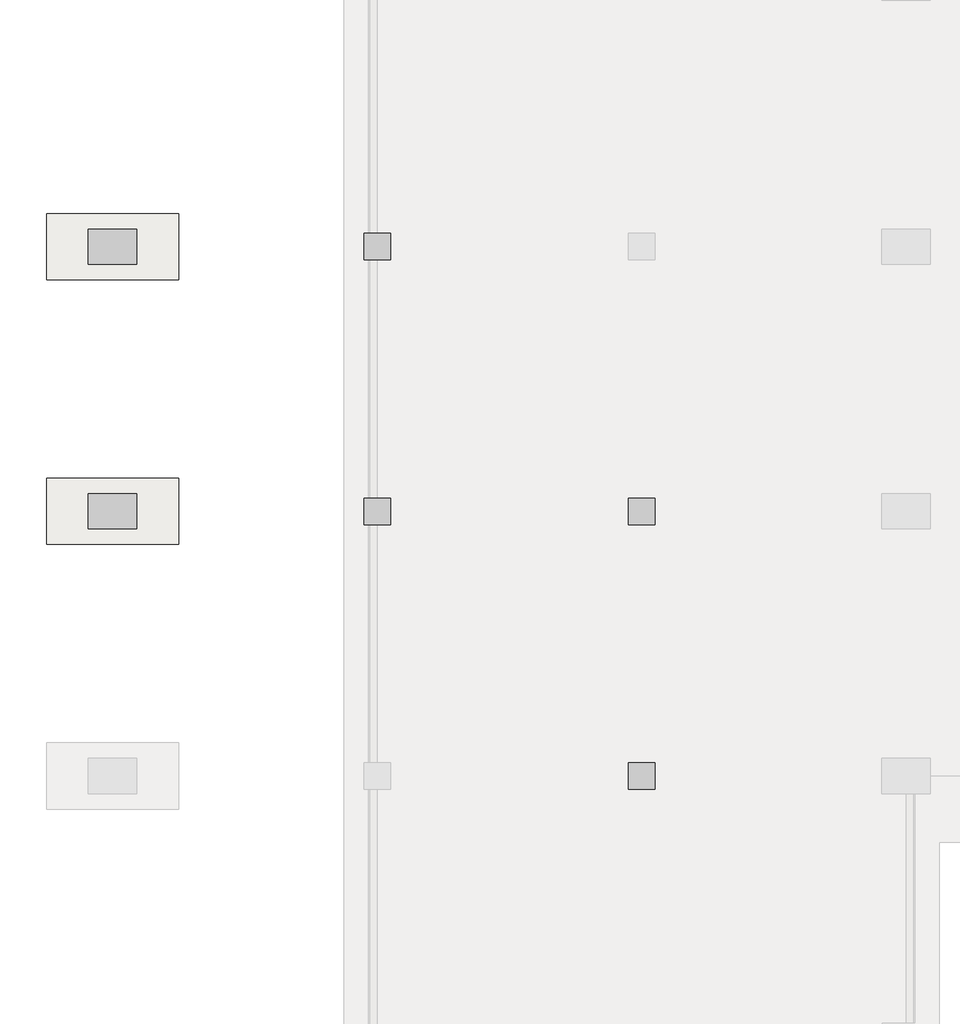
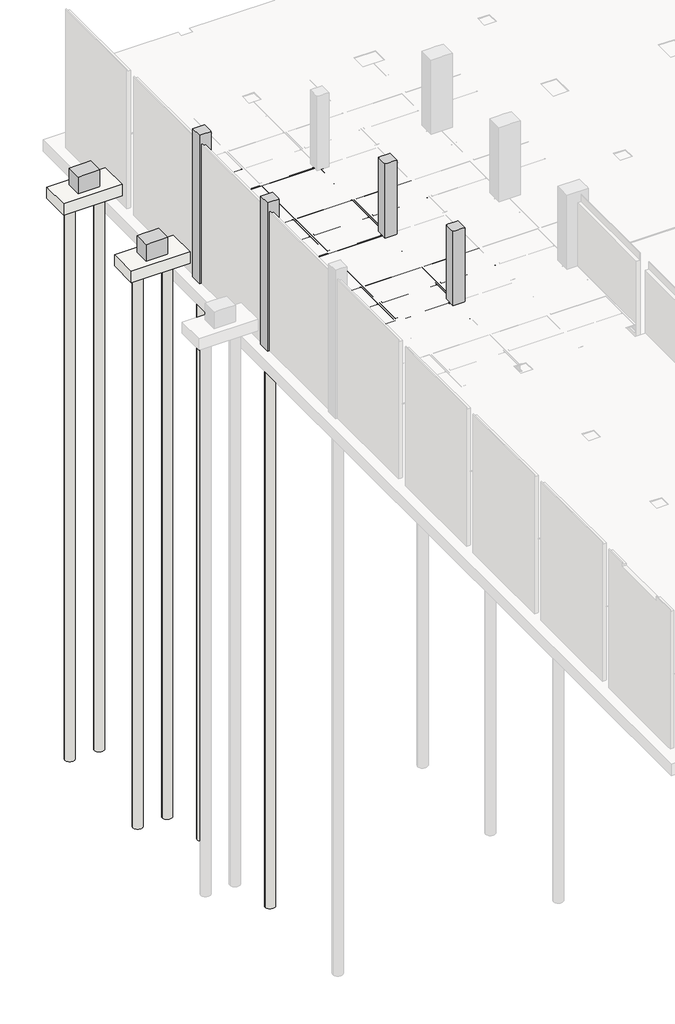
# Not in any storey, part 7 of 16: 27 beams, 8 slabs, 6 columns.
"""IFC4 building model written with IfcOpenShell, lengths in millimetres."""

from ifc_helpers import new_model, si_unit, point, frame, frame_2d, origin, place, context, project, spatial, polyline, circle_curve, trimmed, segment, composite_curve, outline, extrude, faceted_brep, element, save

model = new_model("IFC4")

# Units and contexts
model_context = context("Model", 3, world=origin())
ifc_project = project(units=[si_unit("LENGTHUNIT", "METRE", prefix="MILLI")], contexts=[model_context])

# Site, building
site = spatial("IfcSite", under=ifc_project)
building = spatial("IfcBuilding", under=site)

# Beams
placement = place(None, origin())
element("IfcBeam", 1, ObjectType="Steel Framing_H_KS : H_SB_AR_S02_H-400x200x8x13_BSG1", at=placement, inside=building, context=model_context, shape_type="SweptSolid", body=[
    extrude(outline(composite_curve([segment(polyline([(-17900.0, -4187.0381366), (-17900.0, -4200.0381366), (-18100.0, -4200.0381366), (-18100.0, -4187.0381366), (-18020.0, -4187.0381366)]), True, "CONTINUOUS"), segment(trimmed(circle_curve(frame_2d((-18020.0, -4171.0381366)), 16.0), [point((-18020.0, -4187.0381366))], [point((-18004.0, -4171.0381366))], True, "CARTESIAN"), True, "CONTINUOUS"), segment(polyline([(-18004.0, -4171.0381366), (-18004.0, -3829.0381366)]), True, "CONTINUOUS"), segment(trimmed(circle_curve(frame_2d((-18020.0, -3829.0381366)), 16.0), [point((-18004.0, -3829.0381366))], [point((-18020.0, -3813.0381366))], True, "CARTESIAN"), True, "CONTINUOUS"), segment(polyline([(-18020.0, -3813.0381366), (-18100.0, -3813.0381366), (-18100.0, -3800.0381366), (-17900.0, -3800.0381366), (-17900.0, -3813.0381366), (-17980.0, -3813.0381366)]), True, "CONTINUOUS"), segment(trimmed(circle_curve(frame_2d((-17980.0, -3829.0381366)), 16.0), [point((-17980.0, -3813.0381366))], [point((-17996.0, -3829.0381366))], True, "CARTESIAN"), True, "CONTINUOUS"), segment(polyline([(-17996.0, -3829.0381366), (-17996.0, -4171.0381366)]), True, "CONTINUOUS"), segment(trimmed(circle_curve(frame_2d((-17980.0, -4171.0381366)), 16.0), [point((-17996.0, -4171.0381366))], [point((-17980.0, -4187.0381366))], True, "CARTESIAN"), True, "CONTINUOUS"), segment(polyline([(-17980.0, -4187.0381366), (-17900.0, -4187.0381366)]), True, "CONTINUOUS")], self_intersect=False)), frame((24312.7, 0.0, 0.0), z_axis=(1.0, 0.0, 0.0), x_axis=(0.0, 1.0, 0.0)), (0.0, 0.0, 1.0), 5374.6),
])
element("IfcBeam", 2, ObjectType="Steel Framing_C_KS : H_SB_AR_S02_C-150x75x6.5x10_J1", at=placement, inside=building, context=model_context, shape_type="SweptSolid", body=[
    extrude(outline(composite_curve([segment(polyline([(-16477.2, -3800.0381366), (-16477.2, -3950.0381366), (-16552.2, -3950.0381366)]), True, "CONTINUOUS"), segment(trimmed(circle_curve(frame_2d((-16542.2, -3950.0381366)), 10.0), [point((-16552.2, -3950.0381366))], [point((-16542.2, -3940.0381366))], False, "CARTESIAN"), True, "CONTINUOUS"), segment(polyline([(-16542.2, -3940.0381366), (-16483.7, -3930.7726469), (-16483.7, -3819.3036264), (-16542.2, -3810.0381366)]), True, "CONTINUOUS"), segment(trimmed(circle_curve(frame_2d((-16542.2, -3800.0381366)), 10.0), [point((-16542.2, -3810.0381366))], [point((-16552.2, -3800.0381366))], False, "CARTESIAN"), True, "CONTINUOUS"), segment(polyline([(-16552.2, -3800.0381366), (-16477.2, -3800.0381366)]), True, "CONTINUOUS")], self_intersect=False)), frame((24000.0, 0.0, 0.0), z_axis=(1.0, 0.0, 0.0), x_axis=(0.0, 1.0, 0.0)), (0.0, 0.0, 1.0), 2887.3),
])
element("IfcBeam", 3, ObjectType="Steel Framing_H_KS : H_SB_AR_S02_H-400x200x8x13_BSG1", at=placement, inside=building, context=model_context, shape_type="SweptSolid", body=[
    extrude(outline(composite_curve([segment(polyline([(-23900.0, -4187.0381366), (-23900.0, -4200.0381366), (-24100.0, -4200.0381366), (-24100.0, -4187.0381366), (-24020.0, -4187.0381366)]), True, "CONTINUOUS"), segment(trimmed(circle_curve(frame_2d((-24020.0, -4171.0381366)), 16.0), [point((-24020.0, -4187.0381366))], [point((-24004.0, -4171.0381366))], True, "CARTESIAN"), True, "CONTINUOUS"), segment(polyline([(-24004.0, -4171.0381366), (-24004.0, -3829.0381366)]), True, "CONTINUOUS"), segment(trimmed(circle_curve(frame_2d((-24020.0, -3829.0381366)), 16.0), [point((-24004.0, -3829.0381366))], [point((-24020.0, -3813.0381366))], True, "CARTESIAN"), True, "CONTINUOUS"), segment(polyline([(-24020.0, -3813.0381366), (-24100.0, -3813.0381366), (-24100.0, -3800.0381366), (-23900.0, -3800.0381366), (-23900.0, -3813.0381366), (-23980.0, -3813.0381366)]), True, "CONTINUOUS"), segment(trimmed(circle_curve(frame_2d((-23980.0, -3829.0381366)), 16.0), [point((-23980.0, -3813.0381366))], [point((-23996.0, -3829.0381366))], True, "CARTESIAN"), True, "CONTINUOUS"), segment(polyline([(-23996.0, -3829.0381366), (-23996.0, -4171.0381366)]), True, "CONTINUOUS"), segment(trimmed(circle_curve(frame_2d((-23980.0, -4171.0381366)), 16.0), [point((-23996.0, -4171.0381366))], [point((-23980.0, -4187.0381366))], True, "CARTESIAN"), True, "CONTINUOUS"), segment(polyline([(-23980.0, -4187.0381366), (-23900.0, -4187.0381366)]), True, "CONTINUOUS")], self_intersect=False)), frame((24312.7, 0.0, 0.0), z_axis=(1.0, 0.0, 0.0), x_axis=(0.0, 1.0, 0.0)), (0.0, 0.0, 1.0), 5374.6),
])
element("IfcBeam", 4, ObjectType="Steel Framing_H_KS : H_SB_AR_S02_H-400x200x8x13_BSG2", at=placement, inside=building, context=model_context, shape_type="SweptSolid", body=[
    extrude(outline(composite_curve([segment(polyline([(-4187.0381366, 29900.0), (-4200.0381366, 29900.0), (-4200.0381366, 30100.0), (-4187.0381366, 30100.0), (-4187.0381366, 30020.0)]), True, "CONTINUOUS"), segment(trimmed(circle_curve(frame_2d((-4171.0381366, 30020.0)), 16.0), [point((-4187.0381366, 30020.0))], [point((-4171.0381366, 30004.0))], True, "CARTESIAN"), True, "CONTINUOUS"), segment(polyline([(-4171.0381366, 30004.0), (-3829.0381366, 30004.0)]), True, "CONTINUOUS"), segment(trimmed(circle_curve(frame_2d((-3829.0381366, 30020.0)), 16.0), [point((-3829.0381366, 30004.0))], [point((-3813.0381366, 30020.0))], True, "CARTESIAN"), True, "CONTINUOUS"), segment(polyline([(-3813.0381366, 30020.0), (-3813.0381366, 30100.0), (-3800.0381366, 30100.0), (-3800.0381366, 29900.0), (-3813.0381366, 29900.0), (-3813.0381366, 29980.0)]), True, "CONTINUOUS"), segment(trimmed(circle_curve(frame_2d((-3829.0381366, 29980.0)), 16.0), [point((-3813.0381366, 29980.0))], [point((-3829.0381366, 29996.0))], True, "CARTESIAN"), True, "CONTINUOUS"), segment(polyline([(-3829.0381366, 29996.0), (-4171.0381366, 29996.0)]), True, "CONTINUOUS"), segment(trimmed(circle_curve(frame_2d((-4171.0381366, 29980.0)), 16.0), [point((-4171.0381366, 29996.0))], [point((-4187.0381366, 29980.0))], True, "CARTESIAN"), True, "CONTINUOUS"), segment(polyline([(-4187.0381366, 29980.0), (-4187.0381366, 29900.0)]), True, "CONTINUOUS")], self_intersect=False)), frame((0.0, -23687.3, 0.0), z_axis=(0.0, 1.0, 0.0), x_axis=(0.0, 0.0, 1.0)), (0.0, 0.0, 1.0), 5374.6),
])
element("IfcBeam", 5, ObjectType="Steel Framing_H_KS : H_SB_AR_S02_H-400x200x8x13_BSB1", at=placement, inside=building, context=model_context, shape_type="SweptSolid", body=[
    extrude(outline(composite_curve([segment(polyline([(-4187.0381366, 26900.0), (-4200.0381366, 26900.0), (-4200.0381366, 27100.0), (-4187.0381366, 27100.0), (-4187.0381366, 27020.0)]), True, "CONTINUOUS"), segment(trimmed(circle_curve(frame_2d((-4171.0381366, 27020.0)), 16.0), [point((-4187.0381366, 27020.0))], [point((-4171.0381366, 27004.0))], True, "CARTESIAN"), True, "CONTINUOUS"), segment(polyline([(-4171.0381366, 27004.0), (-3829.0381366, 27004.0)]), True, "CONTINUOUS"), segment(trimmed(circle_curve(frame_2d((-3829.0381366, 27020.0)), 16.0), [point((-3829.0381366, 27004.0))], [point((-3813.0381366, 27020.0))], True, "CARTESIAN"), True, "CONTINUOUS"), segment(polyline([(-3813.0381366, 27020.0), (-3813.0381366, 27100.0), (-3800.0381366, 27100.0), (-3800.0381366, 26900.0), (-3813.0381366, 26900.0), (-3813.0381366, 26980.0)]), True, "CONTINUOUS"), segment(trimmed(circle_curve(frame_2d((-3829.0381366, 26980.0)), 16.0), [point((-3813.0381366, 26980.0))], [point((-3829.0381366, 26996.0))], True, "CARTESIAN"), True, "CONTINUOUS"), segment(polyline([(-3829.0381366, 26996.0), (-4171.0381366, 26996.0)]), True, "CONTINUOUS"), segment(trimmed(circle_curve(frame_2d((-4171.0381366, 26980.0)), 16.0), [point((-4171.0381366, 26996.0))], [point((-4187.0381366, 26980.0))], True, "CARTESIAN"), True, "CONTINUOUS"), segment(polyline([(-4187.0381366, 26980.0), (-4187.0381366, 26900.0)]), True, "CONTINUOUS")], self_intersect=False)), frame((0.0, -23887.3, 0.0), z_axis=(0.0, 1.0, 0.0), x_axis=(0.0, 0.0, 1.0)), (0.0, 0.0, 1.0), 5774.6),
])
element("IfcBeam", 6, ObjectType="Steel Framing_C_KS : H_SB_AR_S02_C-150x75x6.5x10_J1", at=placement, inside=building, context=model_context, shape_type="SweptSolid", body=[
    extrude(outline(composite_curve([segment(polyline([(-20977.2, -3800.0381366), (-20977.2, -3950.0381366), (-21052.2, -3950.0381366)]), True, "CONTINUOUS"), segment(trimmed(circle_curve(frame_2d((-21042.2, -3950.0381366)), 10.0), [point((-21052.2, -3950.0381366))], [point((-21042.2, -3940.0381366))], False, "CARTESIAN"), True, "CONTINUOUS"), segment(polyline([(-21042.2, -3940.0381366), (-20983.7, -3930.7726469), (-20983.7, -3819.3036264), (-21042.2, -3810.0381366)]), True, "CONTINUOUS"), segment(trimmed(circle_curve(frame_2d((-21042.2, -3800.0381366)), 10.0), [point((-21042.2, -3810.0381366))], [point((-21052.2, -3800.0381366))], False, "CARTESIAN"), True, "CONTINUOUS"), segment(polyline([(-21052.2, -3800.0381366), (-20977.2, -3800.0381366)]), True, "CONTINUOUS")], self_intersect=False)), frame((24000.0, 0.0, 0.0), z_axis=(1.0, 0.0, 0.0), x_axis=(0.0, 1.0, 0.0)), (0.0, 0.0, 1.0), 2887.3),
])
element("IfcBeam", 7, ObjectType="Steel Framing_C_KS : H_SB_AR_S02_C-150x75x6.5x10_J1", at=placement, inside=building, context=model_context, shape_type="SweptSolid", body=[
    extrude(outline(composite_curve([segment(polyline([(-22477.2, -3800.0381366), (-22477.2, -3950.0381366), (-22552.2, -3950.0381366)]), True, "CONTINUOUS"), segment(trimmed(circle_curve(frame_2d((-22542.2, -3950.0381366)), 10.0), [point((-22552.2, -3950.0381366))], [point((-22542.2, -3940.0381366))], False, "CARTESIAN"), True, "CONTINUOUS"), segment(polyline([(-22542.2, -3940.0381366), (-22483.7, -3930.7726469), (-22483.7, -3819.3036264), (-22542.2, -3810.0381366)]), True, "CONTINUOUS"), segment(trimmed(circle_curve(frame_2d((-22542.2, -3800.0381366)), 10.0), [point((-22542.2, -3810.0381366))], [point((-22552.2, -3800.0381366))], False, "CARTESIAN"), True, "CONTINUOUS"), segment(polyline([(-22552.2, -3800.0381366), (-22477.2, -3800.0381366)]), True, "CONTINUOUS")], self_intersect=False)), frame((24000.0, 0.0, 0.0), z_axis=(1.0, 0.0, 0.0), x_axis=(0.0, 1.0, 0.0)), (0.0, 0.0, 1.0), 2887.3),
])
element("IfcBeam", 8, ObjectType="Steel Framing_C_KS : H_SB_AR_S02_C-150x75x6.5x10_J1", at=placement, inside=building, context=model_context, shape_type="SweptSolid", body=[
    extrude(outline(composite_curve([segment(polyline([(-19477.2, -3800.0381366), (-19477.2, -3950.0381366), (-19552.2, -3950.0381366)]), True, "CONTINUOUS"), segment(trimmed(circle_curve(frame_2d((-19542.2, -3950.0381366)), 10.0), [point((-19552.2, -3950.0381366))], [point((-19542.2, -3940.0381366))], False, "CARTESIAN"), True, "CONTINUOUS"), segment(polyline([(-19542.2, -3940.0381366), (-19483.7, -3930.7726469), (-19483.7, -3819.3036264), (-19542.2, -3810.0381366)]), True, "CONTINUOUS"), segment(trimmed(circle_curve(frame_2d((-19542.2, -3800.0381366)), 10.0), [point((-19542.2, -3810.0381366))], [point((-19552.2, -3800.0381366))], False, "CARTESIAN"), True, "CONTINUOUS"), segment(polyline([(-19552.2, -3800.0381366), (-19477.2, -3800.0381366)]), True, "CONTINUOUS")], self_intersect=False)), frame((24000.0, 0.0, 0.0), z_axis=(1.0, 0.0, 0.0), x_axis=(0.0, 1.0, 0.0)), (0.0, 0.0, 1.0), 2887.3),
])
element("IfcBeam", 9, ObjectType="Steel Framing_C_KS : H_SB_AR_S02_C-150x75x6.5x10_J1", at=placement, inside=building, context=model_context, shape_type="SweptSolid", body=[
    extrude(outline(composite_curve([segment(polyline([(-20977.2, -3800.0381366), (-20977.2, -3950.0381366), (-21052.2, -3950.0381366)]), True, "CONTINUOUS"), segment(trimmed(circle_curve(frame_2d((-21042.2, -3950.0381366)), 10.0), [point((-21052.2, -3950.0381366))], [point((-21042.2, -3940.0381366))], False, "CARTESIAN"), True, "CONTINUOUS"), segment(polyline([(-21042.2, -3940.0381366), (-20983.7, -3930.7726469), (-20983.7, -3819.3036264), (-21042.2, -3810.0381366)]), True, "CONTINUOUS"), segment(trimmed(circle_curve(frame_2d((-21042.2, -3800.0381366)), 10.0), [point((-21042.2, -3810.0381366))], [point((-21052.2, -3800.0381366))], False, "CARTESIAN"), True, "CONTINUOUS"), segment(polyline([(-21052.2, -3800.0381366), (-20977.2, -3800.0381366)]), True, "CONTINUOUS")], self_intersect=False)), frame((27112.7, 0.0, 0.0), z_axis=(1.0, 0.0, 0.0), x_axis=(0.0, 1.0, 0.0)), (0.0, 0.0, 1.0), 2774.6),
])
element("IfcBeam", 10, ObjectType="Steel Framing_C_KS : H_SB_AR_S02_C-150x75x6.5x10_J1", at=placement, inside=building, context=model_context, shape_type="SweptSolid", body=[
    extrude(outline(composite_curve([segment(polyline([(-22477.2, -3800.0381366), (-22477.2, -3950.0381366), (-22552.2, -3950.0381366)]), True, "CONTINUOUS"), segment(trimmed(circle_curve(frame_2d((-22542.2, -3950.0381366)), 10.0), [point((-22552.2, -3950.0381366))], [point((-22542.2, -3940.0381366))], False, "CARTESIAN"), True, "CONTINUOUS"), segment(polyline([(-22542.2, -3940.0381366), (-22483.7, -3930.7726469), (-22483.7, -3819.3036264), (-22542.2, -3810.0381366)]), True, "CONTINUOUS"), segment(trimmed(circle_curve(frame_2d((-22542.2, -3800.0381366)), 10.0), [point((-22542.2, -3810.0381366))], [point((-22552.2, -3800.0381366))], False, "CARTESIAN"), True, "CONTINUOUS"), segment(polyline([(-22552.2, -3800.0381366), (-22477.2, -3800.0381366)]), True, "CONTINUOUS")], self_intersect=False)), frame((27112.7, 0.0, 0.0), z_axis=(1.0, 0.0, 0.0), x_axis=(0.0, 1.0, 0.0)), (0.0, 0.0, 1.0), 2774.6),
])
element("IfcBeam", 11, ObjectType="Steel Framing_C_KS : H_SB_AR_S02_C-150x75x6.5x10_J1", at=placement, inside=building, context=model_context, shape_type="SweptSolid", body=[
    extrude(outline(composite_curve([segment(polyline([(-19477.2, -3800.0381366), (-19477.2, -3950.0381366), (-19552.2, -3950.0381366)]), True, "CONTINUOUS"), segment(trimmed(circle_curve(frame_2d((-19542.2, -3950.0381366)), 10.0), [point((-19552.2, -3950.0381366))], [point((-19542.2, -3940.0381366))], False, "CARTESIAN"), True, "CONTINUOUS"), segment(polyline([(-19542.2, -3940.0381366), (-19483.7, -3930.7726469), (-19483.7, -3819.3036264), (-19542.2, -3810.0381366)]), True, "CONTINUOUS"), segment(trimmed(circle_curve(frame_2d((-19542.2, -3800.0381366)), 10.0), [point((-19542.2, -3810.0381366))], [point((-19552.2, -3800.0381366))], False, "CARTESIAN"), True, "CONTINUOUS"), segment(polyline([(-19552.2, -3800.0381366), (-19477.2, -3800.0381366)]), True, "CONTINUOUS")], self_intersect=False)), frame((27112.7, 0.0, 0.0), z_axis=(1.0, 0.0, 0.0), x_axis=(0.0, 1.0, 0.0)), (0.0, 0.0, 1.0), 2774.6),
])
element("IfcBeam", 12, ObjectType="Steel Framing_C_KS : H_SB_AR_S02_C-150x75x6.5x10_J1", at=placement, inside=building, context=model_context, shape_type="SweptSolid", body=[
    extrude(outline(composite_curve([segment(polyline([(-20977.2, -3800.0381366), (-20977.2, -3950.0381366), (-21052.2, -3950.0381366)]), True, "CONTINUOUS"), segment(trimmed(circle_curve(frame_2d((-21042.2, -3950.0381366)), 10.0), [point((-21052.2, -3950.0381366))], [point((-21042.2, -3940.0381366))], False, "CARTESIAN"), True, "CONTINUOUS"), segment(polyline([(-21042.2, -3940.0381366), (-20983.7, -3930.7726469), (-20983.7, -3819.3036264), (-21042.2, -3810.0381366)]), True, "CONTINUOUS"), segment(trimmed(circle_curve(frame_2d((-21042.2, -3800.0381366)), 10.0), [point((-21042.2, -3810.0381366))], [point((-21052.2, -3800.0381366))], False, "CARTESIAN"), True, "CONTINUOUS"), segment(polyline([(-21052.2, -3800.0381366), (-20977.2, -3800.0381366)]), True, "CONTINUOUS")], self_intersect=False)), frame((30112.7, 0.0, 0.0), z_axis=(1.0, 0.0, 0.0), x_axis=(0.0, 1.0, 0.0)), (0.0, 0.0, 1.0), 2774.6),
])
element("IfcBeam", 13, ObjectType="Steel Framing_C_KS : H_SB_AR_S02_C-150x75x6.5x10_J1", at=placement, inside=building, context=model_context, shape_type="SweptSolid", body=[
    extrude(outline(composite_curve([segment(polyline([(-22477.2, -3800.0381366), (-22477.2, -3950.0381366), (-22552.2, -3950.0381366)]), True, "CONTINUOUS"), segment(trimmed(circle_curve(frame_2d((-22542.2, -3950.0381366)), 10.0), [point((-22552.2, -3950.0381366))], [point((-22542.2, -3940.0381366))], False, "CARTESIAN"), True, "CONTINUOUS"), segment(polyline([(-22542.2, -3940.0381366), (-22483.7, -3930.7726469), (-22483.7, -3819.3036264), (-22542.2, -3810.0381366)]), True, "CONTINUOUS"), segment(trimmed(circle_curve(frame_2d((-22542.2, -3800.0381366)), 10.0), [point((-22542.2, -3810.0381366))], [point((-22552.2, -3800.0381366))], False, "CARTESIAN"), True, "CONTINUOUS"), segment(polyline([(-22552.2, -3800.0381366), (-22477.2, -3800.0381366)]), True, "CONTINUOUS")], self_intersect=False)), frame((30112.7, 0.0, 0.0), z_axis=(1.0, 0.0, 0.0), x_axis=(0.0, 1.0, 0.0)), (0.0, 0.0, 1.0), 2774.6),
])
element("IfcBeam", 14, ObjectType="Steel Framing_H_KS : H_SB_AR_S02_H-400x200x8x13_BSG1", at=placement, inside=building, context=model_context, shape_type="SweptSolid", body=[
    extrude(outline(composite_curve([segment(polyline([(-29900.0, -4187.0381366), (-29900.0, -4200.0381366), (-30100.0, -4200.0381366), (-30100.0, -4187.0381366), (-30020.0, -4187.0381366)]), True, "CONTINUOUS"), segment(trimmed(circle_curve(frame_2d((-30020.0, -4171.0381366)), 16.0), [point((-30020.0, -4187.0381366))], [point((-30004.0, -4171.0381366))], True, "CARTESIAN"), True, "CONTINUOUS"), segment(polyline([(-30004.0, -4171.0381366), (-30004.0, -3829.0381366)]), True, "CONTINUOUS"), segment(trimmed(circle_curve(frame_2d((-30020.0, -3829.0381366)), 16.0), [point((-30004.0, -3829.0381366))], [point((-30020.0, -3813.0381366))], True, "CARTESIAN"), True, "CONTINUOUS"), segment(polyline([(-30020.0, -3813.0381366), (-30100.0, -3813.0381366), (-30100.0, -3800.0381366), (-29900.0, -3800.0381366), (-29900.0, -3813.0381366), (-29980.0, -3813.0381366)]), True, "CONTINUOUS"), segment(trimmed(circle_curve(frame_2d((-29980.0, -3829.0381366)), 16.0), [point((-29980.0, -3813.0381366))], [point((-29996.0, -3829.0381366))], True, "CARTESIAN"), True, "CONTINUOUS"), segment(polyline([(-29996.0, -3829.0381366), (-29996.0, -4171.0381366)]), True, "CONTINUOUS"), segment(trimmed(circle_curve(frame_2d((-29980.0, -4171.0381366)), 16.0), [point((-29996.0, -4171.0381366))], [point((-29980.0, -4187.0381366))], True, "CARTESIAN"), True, "CONTINUOUS"), segment(polyline([(-29980.0, -4187.0381366), (-29900.0, -4187.0381366)]), True, "CONTINUOUS")], self_intersect=False)), frame((24312.7, 0.0, 0.0), z_axis=(1.0, 0.0, 0.0), x_axis=(0.0, 1.0, 0.0)), (0.0, 0.0, 1.0), 5374.6),
])
element("IfcBeam", 15, ObjectType="Steel Framing_H_KS : H_SB_AR_S02_H-400x200x8x13_BSG2", at=placement, inside=building, context=model_context, shape_type="SweptSolid", body=[
    extrude(outline(composite_curve([segment(polyline([(-4187.0381366, 29900.0), (-4200.0381366, 29900.0), (-4200.0381366, 30100.0), (-4187.0381366, 30100.0), (-4187.0381366, 30020.0)]), True, "CONTINUOUS"), segment(trimmed(circle_curve(frame_2d((-4171.0381366, 30020.0)), 16.0), [point((-4187.0381366, 30020.0))], [point((-4171.0381366, 30004.0))], True, "CARTESIAN"), True, "CONTINUOUS"), segment(polyline([(-4171.0381366, 30004.0), (-3829.0381366, 30004.0)]), True, "CONTINUOUS"), segment(trimmed(circle_curve(frame_2d((-3829.0381366, 30020.0)), 16.0), [point((-3829.0381366, 30004.0))], [point((-3813.0381366, 30020.0))], True, "CARTESIAN"), True, "CONTINUOUS"), segment(polyline([(-3813.0381366, 30020.0), (-3813.0381366, 30100.0), (-3800.0381366, 30100.0), (-3800.0381366, 29900.0), (-3813.0381366, 29900.0), (-3813.0381366, 29980.0)]), True, "CONTINUOUS"), segment(trimmed(circle_curve(frame_2d((-3829.0381366, 29980.0)), 16.0), [point((-3813.0381366, 29980.0))], [point((-3829.0381366, 29996.0))], True, "CARTESIAN"), True, "CONTINUOUS"), segment(polyline([(-3829.0381366, 29996.0), (-4171.0381366, 29996.0)]), True, "CONTINUOUS"), segment(trimmed(circle_curve(frame_2d((-4171.0381366, 29980.0)), 16.0), [point((-4171.0381366, 29996.0))], [point((-4187.0381366, 29980.0))], True, "CARTESIAN"), True, "CONTINUOUS"), segment(polyline([(-4187.0381366, 29980.0), (-4187.0381366, 29900.0)]), True, "CONTINUOUS")], self_intersect=False)), frame((0.0, -29687.3, 0.0), z_axis=(0.0, 1.0, 0.0), x_axis=(0.0, 0.0, 1.0)), (0.0, 0.0, 1.0), 5374.6),
])
element("IfcBeam", 16, ObjectType="Steel Framing_H_KS : H_SB_AR_S02_H-400x200x8x13_BSB1", at=placement, inside=building, context=model_context, shape_type="SweptSolid", body=[
    extrude(outline(composite_curve([segment(polyline([(-4187.0381366, 26900.0), (-4200.0381366, 26900.0), (-4200.0381366, 27100.0), (-4187.0381366, 27100.0), (-4187.0381366, 27020.0)]), True, "CONTINUOUS"), segment(trimmed(circle_curve(frame_2d((-4171.0381366, 27020.0)), 16.0), [point((-4187.0381366, 27020.0))], [point((-4171.0381366, 27004.0))], True, "CARTESIAN"), True, "CONTINUOUS"), segment(polyline([(-4171.0381366, 27004.0), (-3829.0381366, 27004.0)]), True, "CONTINUOUS"), segment(trimmed(circle_curve(frame_2d((-3829.0381366, 27020.0)), 16.0), [point((-3829.0381366, 27004.0))], [point((-3813.0381366, 27020.0))], True, "CARTESIAN"), True, "CONTINUOUS"), segment(polyline([(-3813.0381366, 27020.0), (-3813.0381366, 27100.0), (-3800.0381366, 27100.0), (-3800.0381366, 26900.0), (-3813.0381366, 26900.0), (-3813.0381366, 26980.0)]), True, "CONTINUOUS"), segment(trimmed(circle_curve(frame_2d((-3829.0381366, 26980.0)), 16.0), [point((-3813.0381366, 26980.0))], [point((-3829.0381366, 26996.0))], True, "CARTESIAN"), True, "CONTINUOUS"), segment(polyline([(-3829.0381366, 26996.0), (-4171.0381366, 26996.0)]), True, "CONTINUOUS"), segment(trimmed(circle_curve(frame_2d((-4171.0381366, 26980.0)), 16.0), [point((-4171.0381366, 26996.0))], [point((-4187.0381366, 26980.0))], True, "CARTESIAN"), True, "CONTINUOUS"), segment(polyline([(-4187.0381366, 26980.0), (-4187.0381366, 26900.0)]), True, "CONTINUOUS")], self_intersect=False)), frame((0.0, -29887.3, 0.0), z_axis=(0.0, 1.0, 0.0), x_axis=(0.0, 0.0, 1.0)), (0.0, 0.0, 1.0), 5774.6),
])
element("IfcBeam", 17, ObjectType="Steel Framing_C_KS : H_SB_AR_S02_C-150x75x6.5x10_J1", at=placement, inside=building, context=model_context, shape_type="SweptSolid", body=[
    extrude(outline(composite_curve([segment(polyline([(-26977.2, -3800.0381366), (-26977.2, -3950.0381366), (-27052.2, -3950.0381366)]), True, "CONTINUOUS"), segment(trimmed(circle_curve(frame_2d((-27042.2, -3950.0381366)), 10.0), [point((-27052.2, -3950.0381366))], [point((-27042.2, -3940.0381366))], False, "CARTESIAN"), True, "CONTINUOUS"), segment(polyline([(-27042.2, -3940.0381366), (-26983.7, -3930.7726469), (-26983.7, -3819.3036264), (-27042.2, -3810.0381366)]), True, "CONTINUOUS"), segment(trimmed(circle_curve(frame_2d((-27042.2, -3800.0381366)), 10.0), [point((-27042.2, -3810.0381366))], [point((-27052.2, -3800.0381366))], False, "CARTESIAN"), True, "CONTINUOUS"), segment(polyline([(-27052.2, -3800.0381366), (-26977.2, -3800.0381366)]), True, "CONTINUOUS")], self_intersect=False)), frame((24000.0, 0.0, 0.0), z_axis=(1.0, 0.0, 0.0), x_axis=(0.0, 1.0, 0.0)), (0.0, 0.0, 1.0), 2887.3),
])
element("IfcBeam", 18, ObjectType="Steel Framing_C_KS : H_SB_AR_S02_C-150x75x6.5x10_J1", at=placement, inside=building, context=model_context, shape_type="SweptSolid", body=[
    extrude(outline(composite_curve([segment(polyline([(-28477.2, -3800.0381366), (-28477.2, -3950.0381366), (-28552.2, -3950.0381366)]), True, "CONTINUOUS"), segment(trimmed(circle_curve(frame_2d((-28542.2, -3950.0381366)), 10.0), [point((-28552.2, -3950.0381366))], [point((-28542.2, -3940.0381366))], False, "CARTESIAN"), True, "CONTINUOUS"), segment(polyline([(-28542.2, -3940.0381366), (-28483.7, -3930.7726469), (-28483.7, -3819.3036264), (-28542.2, -3810.0381366)]), True, "CONTINUOUS"), segment(trimmed(circle_curve(frame_2d((-28542.2, -3800.0381366)), 10.0), [point((-28542.2, -3810.0381366))], [point((-28552.2, -3800.0381366))], False, "CARTESIAN"), True, "CONTINUOUS"), segment(polyline([(-28552.2, -3800.0381366), (-28477.2, -3800.0381366)]), True, "CONTINUOUS")], self_intersect=False)), frame((24000.0, 0.0, 0.0), z_axis=(1.0, 0.0, 0.0), x_axis=(0.0, 1.0, 0.0)), (0.0, 0.0, 1.0), 2887.3),
])
element("IfcBeam", 19, ObjectType="Steel Framing_C_KS : H_SB_AR_S02_C-150x75x6.5x10_J1", at=placement, inside=building, context=model_context, shape_type="SweptSolid", body=[
    extrude(outline(composite_curve([segment(polyline([(-25477.2, -3800.0381366), (-25477.2, -3950.0381366), (-25552.2, -3950.0381366)]), True, "CONTINUOUS"), segment(trimmed(circle_curve(frame_2d((-25542.2, -3950.0381366)), 10.0), [point((-25552.2, -3950.0381366))], [point((-25542.2, -3940.0381366))], False, "CARTESIAN"), True, "CONTINUOUS"), segment(polyline([(-25542.2, -3940.0381366), (-25483.7, -3930.7726469), (-25483.7, -3819.3036264), (-25542.2, -3810.0381366)]), True, "CONTINUOUS"), segment(trimmed(circle_curve(frame_2d((-25542.2, -3800.0381366)), 10.0), [point((-25542.2, -3810.0381366))], [point((-25552.2, -3800.0381366))], False, "CARTESIAN"), True, "CONTINUOUS"), segment(polyline([(-25552.2, -3800.0381366), (-25477.2, -3800.0381366)]), True, "CONTINUOUS")], self_intersect=False)), frame((24000.0, 0.0, 0.0), z_axis=(1.0, 0.0, 0.0), x_axis=(0.0, 1.0, 0.0)), (0.0, 0.0, 1.0), 2887.3),
])
element("IfcBeam", 20, ObjectType="Steel Framing_C_KS : H_SB_AR_S02_C-150x75x6.5x10_J1", at=placement, inside=building, context=model_context, shape_type="SweptSolid", body=[
    extrude(outline(composite_curve([segment(polyline([(-26977.2, -3800.0381366), (-26977.2, -3950.0381366), (-27052.2, -3950.0381366)]), True, "CONTINUOUS"), segment(trimmed(circle_curve(frame_2d((-27042.2, -3950.0381366)), 10.0), [point((-27052.2, -3950.0381366))], [point((-27042.2, -3940.0381366))], False, "CARTESIAN"), True, "CONTINUOUS"), segment(polyline([(-27042.2, -3940.0381366), (-26983.7, -3930.7726469), (-26983.7, -3819.3036264), (-27042.2, -3810.0381366)]), True, "CONTINUOUS"), segment(trimmed(circle_curve(frame_2d((-27042.2, -3800.0381366)), 10.0), [point((-27042.2, -3810.0381366))], [point((-27052.2, -3800.0381366))], False, "CARTESIAN"), True, "CONTINUOUS"), segment(polyline([(-27052.2, -3800.0381366), (-26977.2, -3800.0381366)]), True, "CONTINUOUS")], self_intersect=False)), frame((27112.7, 0.0, 0.0), z_axis=(1.0, 0.0, 0.0), x_axis=(0.0, 1.0, 0.0)), (0.0, 0.0, 1.0), 2774.6),
])
element("IfcBeam", 21, ObjectType="Steel Framing_C_KS : H_SB_AR_S02_C-150x75x6.5x10_J1", at=placement, inside=building, context=model_context, shape_type="SweptSolid", body=[
    extrude(outline(composite_curve([segment(polyline([(-28477.2, -3800.0381366), (-28477.2, -3950.0381366), (-28552.2, -3950.0381366)]), True, "CONTINUOUS"), segment(trimmed(circle_curve(frame_2d((-28542.2, -3950.0381366)), 10.0), [point((-28552.2, -3950.0381366))], [point((-28542.2, -3940.0381366))], False, "CARTESIAN"), True, "CONTINUOUS"), segment(polyline([(-28542.2, -3940.0381366), (-28483.7, -3930.7726469), (-28483.7, -3819.3036264), (-28542.2, -3810.0381366)]), True, "CONTINUOUS"), segment(trimmed(circle_curve(frame_2d((-28542.2, -3800.0381366)), 10.0), [point((-28542.2, -3810.0381366))], [point((-28552.2, -3800.0381366))], False, "CARTESIAN"), True, "CONTINUOUS"), segment(polyline([(-28552.2, -3800.0381366), (-28477.2, -3800.0381366)]), True, "CONTINUOUS")], self_intersect=False)), frame((27112.7, 0.0, 0.0), z_axis=(1.0, 0.0, 0.0), x_axis=(0.0, 1.0, 0.0)), (0.0, 0.0, 1.0), 2774.6),
])
element("IfcBeam", 22, ObjectType="Steel Framing_C_KS : H_SB_AR_S02_C-150x75x6.5x10_J1", at=placement, inside=building, context=model_context, shape_type="SweptSolid", body=[
    extrude(outline(composite_curve([segment(polyline([(-25477.2, -3800.0381366), (-25477.2, -3950.0381366), (-25552.2, -3950.0381366)]), True, "CONTINUOUS"), segment(trimmed(circle_curve(frame_2d((-25542.2, -3950.0381366)), 10.0), [point((-25552.2, -3950.0381366))], [point((-25542.2, -3940.0381366))], False, "CARTESIAN"), True, "CONTINUOUS"), segment(polyline([(-25542.2, -3940.0381366), (-25483.7, -3930.7726469), (-25483.7, -3819.3036264), (-25542.2, -3810.0381366)]), True, "CONTINUOUS"), segment(trimmed(circle_curve(frame_2d((-25542.2, -3800.0381366)), 10.0), [point((-25542.2, -3810.0381366))], [point((-25552.2, -3800.0381366))], False, "CARTESIAN"), True, "CONTINUOUS"), segment(polyline([(-25552.2, -3800.0381366), (-25477.2, -3800.0381366)]), True, "CONTINUOUS")], self_intersect=False)), frame((27112.7, 0.0, 0.0), z_axis=(1.0, 0.0, 0.0), x_axis=(0.0, 1.0, 0.0)), (0.0, 0.0, 1.0), 2774.6),
])
element("IfcBeam", 23, ObjectType="Steel Framing_C_KS : H_SB_AR_S02_C-150x75x6.5x10_J1", at=placement, inside=building, context=model_context, shape_type="SweptSolid", body=[
    extrude(outline(composite_curve([segment(polyline([(-26977.2, -3800.0381366), (-26977.2, -3950.0381366), (-27052.2, -3950.0381366)]), True, "CONTINUOUS"), segment(trimmed(circle_curve(frame_2d((-27042.2, -3950.0381366)), 10.0), [point((-27052.2, -3950.0381366))], [point((-27042.2, -3940.0381366))], False, "CARTESIAN"), True, "CONTINUOUS"), segment(polyline([(-27042.2, -3940.0381366), (-26983.7, -3930.7726469), (-26983.7, -3819.3036264), (-27042.2, -3810.0381366)]), True, "CONTINUOUS"), segment(trimmed(circle_curve(frame_2d((-27042.2, -3800.0381366)), 10.0), [point((-27042.2, -3810.0381366))], [point((-27052.2, -3800.0381366))], False, "CARTESIAN"), True, "CONTINUOUS"), segment(polyline([(-27052.2, -3800.0381366), (-26977.2, -3800.0381366)]), True, "CONTINUOUS")], self_intersect=False)), frame((30112.7, 0.0, 0.0), z_axis=(1.0, 0.0, 0.0), x_axis=(0.0, 1.0, 0.0)), (0.0, 0.0, 1.0), 2774.6),
])
element("IfcBeam", 24, ObjectType="Steel Framing_C_KS : H_SB_AR_S02_C-150x75x6.5x10_J1", at=placement, inside=building, context=model_context, shape_type="SweptSolid", body=[
    extrude(outline(composite_curve([segment(polyline([(-28477.2, -3800.0381366), (-28477.2, -3950.0381366), (-28552.2, -3950.0381366)]), True, "CONTINUOUS"), segment(trimmed(circle_curve(frame_2d((-28542.2, -3950.0381366)), 10.0), [point((-28552.2, -3950.0381366))], [point((-28542.2, -3940.0381366))], False, "CARTESIAN"), True, "CONTINUOUS"), segment(polyline([(-28542.2, -3940.0381366), (-28483.7, -3930.7726469), (-28483.7, -3819.3036264), (-28542.2, -3810.0381366)]), True, "CONTINUOUS"), segment(trimmed(circle_curve(frame_2d((-28542.2, -3800.0381366)), 10.0), [point((-28542.2, -3810.0381366))], [point((-28552.2, -3800.0381366))], False, "CARTESIAN"), True, "CONTINUOUS"), segment(polyline([(-28552.2, -3800.0381366), (-28477.2, -3800.0381366)]), True, "CONTINUOUS")], self_intersect=False)), frame((30112.7, 0.0, 0.0), z_axis=(1.0, 0.0, 0.0), x_axis=(0.0, 1.0, 0.0)), (0.0, 0.0, 1.0), 2774.6),
])
element("IfcBeam", 25, ObjectType="Steel Framing_C_KS : H_SB_AR_S02_C-150x75x6.5x10_J1", at=placement, inside=building, context=model_context, shape_type="SweptSolid", body=[
    extrude(outline(composite_curve([segment(polyline([(-25477.2, -3800.0381366), (-25477.2, -3950.0381366), (-25552.2, -3950.0381366)]), True, "CONTINUOUS"), segment(trimmed(circle_curve(frame_2d((-25542.2, -3950.0381366)), 10.0), [point((-25552.2, -3950.0381366))], [point((-25542.2, -3940.0381366))], False, "CARTESIAN"), True, "CONTINUOUS"), segment(polyline([(-25542.2, -3940.0381366), (-25483.7, -3930.7726469), (-25483.7, -3819.3036264), (-25542.2, -3810.0381366)]), True, "CONTINUOUS"), segment(trimmed(circle_curve(frame_2d((-25542.2, -3800.0381366)), 10.0), [point((-25542.2, -3810.0381366))], [point((-25552.2, -3800.0381366))], False, "CARTESIAN"), True, "CONTINUOUS"), segment(polyline([(-25552.2, -3800.0381366), (-25477.2, -3800.0381366)]), True, "CONTINUOUS")], self_intersect=False)), frame((30112.7, 0.0, 0.0), z_axis=(1.0, 0.0, 0.0), x_axis=(0.0, 1.0, 0.0)), (0.0, 0.0, 1.0), 2774.6),
])
element("IfcBeam", 26, ObjectType="Steel Framing_C_KS : H_SB_AR_S02_C-150x75x6.5x10_J1", at=placement, inside=building, context=model_context, shape_type="SweptSolid", body=[
    extrude(outline(composite_curve([segment(polyline([(-31477.2, -3800.0381366), (-31477.2, -3950.0381366), (-31552.2, -3950.0381366)]), True, "CONTINUOUS"), segment(trimmed(circle_curve(frame_2d((-31542.2, -3950.0381366)), 10.0), [point((-31552.2, -3950.0381366))], [point((-31542.2, -3940.0381366))], False, "CARTESIAN"), True, "CONTINUOUS"), segment(polyline([(-31542.2, -3940.0381366), (-31483.7, -3930.7726469), (-31483.7, -3819.3036264), (-31542.2, -3810.0381366)]), True, "CONTINUOUS"), segment(trimmed(circle_curve(frame_2d((-31542.2, -3800.0381366)), 10.0), [point((-31542.2, -3810.0381366))], [point((-31552.2, -3800.0381366))], False, "CARTESIAN"), True, "CONTINUOUS"), segment(polyline([(-31552.2, -3800.0381366), (-31477.2, -3800.0381366)]), True, "CONTINUOUS")], self_intersect=False)), frame((27112.7, 0.0, 0.0), z_axis=(1.0, 0.0, 0.0), x_axis=(0.0, 1.0, 0.0)), (0.0, 0.0, 1.0), 2774.6),
])
element("IfcBeam", 27, ObjectType="Steel Framing_C_KS : H_SB_AR_S02_C-150x75x6.5x10_J1", at=placement, inside=building, context=model_context, shape_type="SweptSolid", body=[
    extrude(outline(composite_curve([segment(polyline([(-31477.2, -3800.0381366), (-31477.2, -3950.0381366), (-31552.2, -3950.0381366)]), True, "CONTINUOUS"), segment(trimmed(circle_curve(frame_2d((-31542.2, -3950.0381366)), 10.0), [point((-31552.2, -3950.0381366))], [point((-31542.2, -3940.0381366))], False, "CARTESIAN"), True, "CONTINUOUS"), segment(polyline([(-31542.2, -3940.0381366), (-31483.7, -3930.7726469), (-31483.7, -3819.3036264), (-31542.2, -3810.0381366)]), True, "CONTINUOUS"), segment(trimmed(circle_curve(frame_2d((-31542.2, -3800.0381366)), 10.0), [point((-31542.2, -3810.0381366))], [point((-31552.2, -3800.0381366))], False, "CARTESIAN"), True, "CONTINUOUS"), segment(polyline([(-31552.2, -3800.0381366), (-31477.2, -3800.0381366)]), True, "CONTINUOUS")], self_intersect=False)), frame((30112.7, 0.0, 0.0), z_axis=(1.0, 0.0, 0.0), x_axis=(0.0, 1.0, 0.0)), (0.0, 0.0, 1.0), 2774.6),
])

# Columns
element("IfcColumn", 28, ObjectType="RC_Column_Rectangular : H_SC_AR_S15_UG PED_Bit_800x1100_PD1", at=placement, inside=building, context=model_context, shape_type="Brep", body=[
    faceted_brep([(17450.0, -17600.0, -700.0381366), (18550.0, -17600.0, -700.0381366), (18550.0, -18400.0, -700.0381366), (17450.0, -18400.0, -700.0381366), (17450.0, -17600.0, 199.9618634), (17800.0, -17600.0, 199.9618634), (18200.0, -17600.0, 199.9618634), (18550.0, -17600.0, 199.9618634), (18550.0, -17600.0, -0.0381366), (17450.0, -17600.0, -0.0381366), (18550.0, -18400.0, 199.9618634), (18550.0, -18400.0, -0.0381366), (18200.0, -18400.0, 199.9618634), (17800.0, -18400.0, 199.9618634), (17450.0, -18400.0, 199.9618634), (17450.0, -18400.0, -0.0381366)], [[[0, 1, 2, 3]], [[4, 5, 6, 7, 8, 1, 0, 9]], [[7, 10, 11, 2, 1, 8]], [[10, 12, 13, 14, 15, 3, 2, 11]], [[14, 4, 9, 0, 3, 15]], [[4, 14, 13, 12, 10, 7, 6, 5]]]),
])
element("IfcColumn", 29, ObjectType="RC_Column_Rectangular : H_SC_AR_S15_UG PED_Bit_800x1100_PD1", at=placement, inside=building, context=model_context, shape_type="Brep", body=[
    faceted_brep([(17450.0, -23600.0, -700.0381366), (18550.0, -23600.0, -700.0381366), (18550.0, -24400.0, -700.0381366), (17450.0, -24400.0, -700.0381366), (17450.0, -23600.0, 199.9618634), (17800.0, -23600.0, 199.9618634), (18200.0, -23600.0, 199.9618634), (18550.0, -23600.0, 199.9618634), (18550.0, -23600.0, -0.0381366), (17450.0, -23600.0, -0.0381366), (18550.0, -24400.0, 199.9618634), (18550.0, -24400.0, -0.0381366), (18200.0, -24400.0, 199.9618634), (17800.0, -24400.0, 199.9618634), (17450.0, -24400.0, 199.9618634), (17450.0, -24400.0, -0.0381366)], [[[0, 1, 2, 3]], [[4, 5, 6, 7, 8, 1, 0, 9]], [[7, 10, 11, 2, 1, 8]], [[10, 12, 13, 14, 15, 3, 2, 11]], [[14, 4, 9, 0, 3, 15]], [[4, 14, 13, 12, 10, 7, 6, 5]]]),
])
element("IfcColumn", 30, ObjectType="RC_Column_Rectangular : H_SC_AR_S15_UG PED_Bit_600x600_BC1", at=placement, inside=building, context=model_context, shape_type="Brep", body=[
    faceted_brep([(30300.0, -23700.0, -7200.0381366), (30300.0, -24300.0, -7200.0381366), (29700.0, -24300.0, -7200.0381366), (29700.0, -23700.0, -7200.0381366), (30300.0, -23700.0, 199.9618634), (30300.0, -23825.0, 199.9618634), (30300.0, -24175.0, 199.9618634), (30300.0, -24300.0, 199.9618634), (30300.0, -24300.0, 167.9618634), (30300.0, -24300.0, -3800.0381366), (30300.0, -24300.0, -3832.0381366), (30300.0, -23700.0, -3832.0381366), (30300.0, -23700.0, -3800.0381366), (30300.0, -23700.0, 167.9618634), (30175.0, -24300.0, 199.9618634), (29825.0, -24300.0, 199.9618634), (29700.0, -24300.0, 199.9618634), (29700.0, -24300.0, -0.0381366), (29700.0, -24300.0, -3800.0381366), (29700.0, -24300.0, -3832.0381366), (29700.0, -24175.0, 199.9618634), (29700.0, -23825.0, 199.9618634), (29700.0, -23700.0, 199.9618634), (29700.0, -23700.0, -0.0381366), (29700.0, -23700.0, -3800.0381366), (29700.0, -23700.0, -3832.0381366), (29825.0, -23700.0, 199.9618634), (30175.0, -23700.0, 199.9618634)], [[[0, 1, 2, 3]], [[4, 5, 6, 7, 8, 9, 10, 1, 0, 11, 12, 13]], [[7, 14, 15, 16, 17, 18, 19, 2, 1, 10, 9, 8]], [[16, 20, 21, 22, 23, 24, 25, 3, 2, 19, 18, 17]], [[22, 26, 27, 4, 13, 12, 11, 0, 3, 25, 24, 23]], [[4, 27, 26, 22, 21, 20, 16, 15, 14, 7, 6, 5]]]),
])
element("IfcColumn", 31, ObjectType="RC_Column_Rectangular : H_SC_AR_S15_UG PED_Bit_600x600_BC1", at=placement, inside=building, context=model_context, shape_type="Brep", body=[
    faceted_brep([(24300.0, -23700.0, -7800.0381366), (24300.0, -24300.0, -7800.0381366), (24000.0, -24300.0, -7800.0381366), (23800.0, -24300.0, -7800.0381366), (23700.0, -24300.0, -7800.0381366), (23700.0, -23700.0, -7800.0381366), (23800.0, -23700.0, -7800.0381366), (24000.0, -23700.0, -7800.0381366), (24300.0, -23700.0, 199.9618634), (24300.0, -23825.0, 199.9618634), (24300.0, -24175.0, 199.9618634), (24300.0, -24300.0, 199.9618634), (24300.0, -24300.0, -0.0381366), (24300.0, -24300.0, -3800.0381366), (24300.0, -24300.0, -3832.0381366), (24300.0, -23700.0, -3832.0381366), (24300.0, -23700.0, -3800.0381366), (24300.0, -23700.0, -0.0381366), (24000.0, -24300.0, 199.9618634), (23700.0, -24300.0, 199.9618634), (23700.0, -24300.0, -0.0381366), (23700.0, -23700.0, 199.9618634), (23700.0, -23700.0, -0.0381366), (24000.0, -23700.0, 199.9618634)], [[[0, 1, 2, 3, 4, 5, 6, 7]], [[8, 9, 10, 11, 12, 13, 14, 1, 0, 15, 16, 17]], [[11, 18, 19, 20, 4, 3, 2, 1, 14, 13, 12]], [[19, 21, 22, 5, 4, 20]], [[21, 23, 8, 17, 16, 15, 0, 7, 6, 5, 22]], [[8, 23, 21, 19, 18, 11, 10, 9]]]),
])
element("IfcColumn", 32, ObjectType="RC_Column_Rectangular : H_SC_AR_S15_UG PED_Bit_600x600_BC1", at=placement, inside=building, context=model_context, shape_type="Brep", body=[
    faceted_brep([(24300.0, -17700.0, -7800.0381366), (24300.0, -18300.0, -7800.0381366), (24000.0, -18300.0, -7800.0381366), (23800.0, -18300.0, -7800.0381366), (23700.0, -18300.0, -7800.0381366), (23700.0, -17700.0, -7800.0381366), (23800.0, -17700.0, -7800.0381366), (24000.0, -17700.0, -7800.0381366), (24300.0, -17700.0, 199.9618634), (24300.0, -17825.0, 199.9618634), (24300.0, -18175.0, 199.9618634), (24300.0, -18300.0, 199.9618634), (24300.0, -18300.0, -0.0381366), (24300.0, -18300.0, -3800.0381366), (24300.0, -18300.0, -3832.0381366), (24300.0, -17700.0, -3832.0381366), (24300.0, -17700.0, -3800.0381366), (24300.0, -17700.0, -0.0381366), (24000.0, -18300.0, 199.9618634), (23700.0, -18300.0, 199.9618634), (23700.0, -18300.0, -0.0381366), (23700.0, -17700.0, 199.9618634), (23700.0, -17700.0, -0.0381366), (24000.0, -17700.0, 199.9618634)], [[[0, 1, 2, 3, 4, 5, 6, 7]], [[8, 9, 10, 11, 12, 13, 14, 1, 0, 15, 16, 17]], [[11, 18, 19, 20, 4, 3, 2, 1, 14, 13, 12]], [[19, 21, 22, 5, 4, 20]], [[21, 23, 8, 17, 16, 15, 0, 7, 6, 5, 22]], [[8, 23, 21, 19, 18, 11, 10, 9]]]),
])
element("IfcColumn", 33, ObjectType="RC_Column_Rectangular : H_SC_AR_S15_UG PED_Bit_600x600_BC1", at=placement, inside=building, context=model_context, shape_type="Brep", body=[
    faceted_brep([(30300.0, -29700.0, -7200.0381366), (30300.0, -30300.0, -7200.0381366), (29700.0, -30300.0, -7200.0381366), (29700.0, -29700.0, -7200.0381366), (30300.0, -29700.0, 199.9618634), (30300.0, -29825.0, 199.9618634), (30300.0, -30175.0, 199.9618634), (30300.0, -30300.0, 199.9618634), (30300.0, -30300.0, 167.9618634), (30300.0, -30300.0, -3800.0381366), (30300.0, -30300.0, -3832.0381366), (30300.0, -29700.0, -3832.0381366), (30300.0, -29700.0, -3800.0381366), (30300.0, -29700.0, 167.9618634), (30175.0, -30300.0, 199.9618634), (29825.0, -30300.0, 199.9618634), (29700.0, -30300.0, 199.9618634), (29700.0, -30300.0, -0.0381366), (29700.0, -30300.0, -3800.0381366), (29700.0, -30300.0, -3832.0381366), (29700.0, -30175.0, 199.9618634), (29700.0, -29825.0, 199.9618634), (29700.0, -29700.0, 199.9618634), (29700.0, -29700.0, -0.0381366), (29700.0, -29700.0, -3800.0381366), (29700.0, -29700.0, -3832.0381366), (29825.0, -29700.0, 199.9618634), (30175.0, -29700.0, 199.9618634)], [[[0, 1, 2, 3]], [[4, 5, 6, 7, 8, 9, 10, 1, 0, 11, 12, 13]], [[7, 14, 15, 16, 17, 18, 19, 2, 1, 10, 9, 8]], [[16, 20, 21, 22, 23, 24, 25, 3, 2, 19, 18, 17]], [[22, 26, 27, 4, 13, 12, 11, 0, 3, 25, 24, 23]], [[4, 27, 26, 22, 21, 20, 16, 15, 14, 7, 6, 5]]]),
])

# Slabs
element("IfcSlab", 34, ObjectType="Foundation Rectangular (Non-Pile) : H_SF_AR_S18_Shallow Fdn_Bitumen_1500x3000xT600_F1", at=placement, inside=building, context=model_context, shape_type="SweptSolid", body=[
    extrude(outline(polyline([(19500.0, -18750.0), (16500.0, -18750.0), (16500.0, -17250.0), (19500.0, -17250.0), (19500.0, -18750.0)])), frame((0.0, 0.0, -1300.0381366), z_axis=(0.0, 0.0, 1.0), x_axis=(1.0, 0.0, 0.0)), (0.0, 0.0, 1.0), 600.0),
])
element("IfcSlab", 35, ObjectType="Foundation Rectangular (Non-Pile) : H_SF_AR_S18_Shallow Fdn_Bitumen_1500x3000xT600_F1", at=placement, inside=building, context=model_context, shape_type="SweptSolid", body=[
    extrude(outline(polyline([(19500.0, -24750.0), (16500.0, -24750.0), (16500.0, -23250.0), (19500.0, -23250.0), (19500.0, -24750.0)])), frame((0.0, 0.0, -1300.0381366), z_axis=(0.0, 0.0, 1.0), x_axis=(1.0, 0.0, 0.0)), (0.0, 0.0, 1.0), 600.0),
])
element("IfcSlab", 36, ObjectType="PILE : H_SF_AR_S19_PHC Pile_Pre-boring_D500_L30", at=placement, inside=building, context=model_context, shape_type="SweptSolid", body=[
    extrude(outline(composite_curve([segment(trimmed(circle_curve(frame_2d((17250.0, -24000.0)), 250.0), [point((17000.0, -24000.0))], [point((17500.0, -24000.0))], False, "CARTESIAN"), True, "CONTINUOUS"), segment(trimmed(circle_curve(frame_2d((17250.0, -24000.0)), 250.0), [point((17500.0, -24000.0))], [point((17000.0, -24000.0))], False, "CARTESIAN"), True, "CONTINUOUS")], self_intersect=False)), frame((0.0, 0.0, -31300.0381366), z_axis=(0.0, 0.0, 1.0), x_axis=(1.0, 0.0, 0.0)), (0.0, 0.0, 1.0), 30000.0),
])
element("IfcSlab", 37, ObjectType="PILE : H_SF_AR_S19_PHC Pile_Pre-boring_D500_L30", at=placement, inside=building, context=model_context, shape_type="SweptSolid", body=[
    extrude(outline(composite_curve([segment(trimmed(circle_curve(frame_2d((18750.0, -24000.0)), 250.0), [point((18500.0, -24000.0))], [point((19000.0, -24000.0))], False, "CARTESIAN"), True, "CONTINUOUS"), segment(trimmed(circle_curve(frame_2d((18750.0, -24000.0)), 250.0), [point((19000.0, -24000.0))], [point((18500.0, -24000.0))], False, "CARTESIAN"), True, "CONTINUOUS")], self_intersect=False)), frame((0.0, 0.0, -31300.0381366), z_axis=(0.0, 0.0, 1.0), x_axis=(1.0, 0.0, 0.0)), (0.0, 0.0, 1.0), 30000.0),
])
element("IfcSlab", 38, ObjectType="PILE : H_SF_AR_S19_PHC Pile_Pre-boring_D500_L30", at=placement, inside=building, context=model_context, shape_type="SweptSolid", body=[
    extrude(outline(composite_curve([segment(trimmed(circle_curve(frame_2d((17250.0, -18000.0)), 250.0), [point((17000.0, -18000.0))], [point((17500.0, -18000.0))], False, "CARTESIAN"), True, "CONTINUOUS"), segment(trimmed(circle_curve(frame_2d((17250.0, -18000.0)), 250.0), [point((17500.0, -18000.0))], [point((17000.0, -18000.0))], False, "CARTESIAN"), True, "CONTINUOUS")], self_intersect=False)), frame((0.0, 0.0, -31300.0381366), z_axis=(0.0, 0.0, 1.0), x_axis=(1.0, 0.0, 0.0)), (0.0, 0.0, 1.0), 30000.0),
])
element("IfcSlab", 39, ObjectType="PILE : H_SF_AR_S19_PHC Pile_Pre-boring_D500_L30", at=placement, inside=building, context=model_context, shape_type="SweptSolid", body=[
    extrude(outline(composite_curve([segment(trimmed(circle_curve(frame_2d((18750.0, -18000.0)), 250.0), [point((18500.0, -18000.0))], [point((19000.0, -18000.0))], False, "CARTESIAN"), True, "CONTINUOUS"), segment(trimmed(circle_curve(frame_2d((18750.0, -18000.0)), 250.0), [point((19000.0, -18000.0))], [point((18500.0, -18000.0))], False, "CARTESIAN"), True, "CONTINUOUS")], self_intersect=False)), frame((0.0, 0.0, -31300.0381366), z_axis=(0.0, 0.0, 1.0), x_axis=(1.0, 0.0, 0.0)), (0.0, 0.0, 1.0), 30000.0),
])
element("IfcSlab", 40, ObjectType="PILE : H_SF_AR_S19_PHC Pile_Pre-boring_D500_L30", at=placement, inside=building, context=model_context, shape_type="SweptSolid", body=[
    extrude(outline(composite_curve([segment(trimmed(circle_curve(frame_2d((24000.0, -24000.0)), 250.0), [point((23750.0, -24000.0))], [point((24250.0, -24000.0))], False, "CARTESIAN"), True, "CONTINUOUS"), segment(trimmed(circle_curve(frame_2d((24000.0, -24000.0)), 250.0), [point((24250.0, -24000.0))], [point((23750.0, -24000.0))], False, "CARTESIAN"), True, "CONTINUOUS")], self_intersect=False)), frame((0.0, 0.0, -37950.0381366), z_axis=(0.0, 0.0, 1.0), x_axis=(1.0, 0.0, 0.0)), (0.0, 0.0, 1.0), 29550.0),
])
element("IfcSlab", 41, ObjectType="PILE : H_SF_AR_S19_PHC Pile_Pre-boring_D500_L30", at=placement, inside=building, context=model_context, shape_type="SweptSolid", body=[
    extrude(outline(composite_curve([segment(trimmed(circle_curve(frame_2d((24000.0, -18000.0)), 250.0), [point((23750.0, -18000.0))], [point((24250.0, -18000.0))], False, "CARTESIAN"), True, "CONTINUOUS"), segment(trimmed(circle_curve(frame_2d((24000.0, -18000.0)), 250.0), [point((24250.0, -18000.0))], [point((23750.0, -18000.0))], False, "CARTESIAN"), True, "CONTINUOUS")], self_intersect=False)), frame((0.0, 0.0, -37950.0381366), z_axis=(0.0, 0.0, 1.0), x_axis=(1.0, 0.0, 0.0)), (0.0, 0.0, 1.0), 29550.0),
])

save(model, "model.ifc")

# Revit data of these elements
# Type "Steel Framing_H_KS : H_SB_AR_S02_H-400x200x8x13_BSG1"
#   Type Comments = "MAIN"
#   Type Mark = "BSG1"
#   H_SectionID = "H-400x200x8x13"
#   H_Ratio for Additional Steel Plate = 0.2
#   Width = 20.0 cm
#   Web Thickness = 0.8 cm
#   Web Fillet = 1.6 cm
#   Warping Constant = 649000.0 cm⁶
#   Torsional Moment of Inertia = 35.8981 cm⁴
#   Section Area = 84.12 cm²
#   Plastic Modulus weak axis = 268.0 cm³
#   Plastic Modulus strong axis = 1330.0 cm³
#   Perimeter = 1.56 m²/m
#   Nominal Weight = 66.00 kgf/m
#   Moment of Inertia weak axis = 1740.00 cm⁴
#   Moment of Inertia strong axis = 23700.00 cm⁴
#   Height = 40.0 cm
#   Flange Thickness = 1.3 cm
#   Elastic Modulus weak axis = 174.0 cm³
#   Elastic Modulus strong axis = 1190.0 cm³
#   Centroid Vertical = 20.0 cm
#   Centroid Horizontal = 10.0 cm
#   Bolt Spacing = 8.89 cm
#   Length [instance default] = 1500 mm
#   Structural Material [instance default] = Steel, 45-345
#   Section Name Key = ""
#   Assembly Code = ""
# Type "Steel Framing_C_KS : H_SB_AR_S02_C-150x75x6.5x10_J1"
#   Type Mark = "J1"
#   H_SectionID = "C-150x75x6.5x10"
#   Assembly Code = "B10"
#   H_Ratio for Additional Steel Plate = 0.2
#   Perimeter = 0.51 m²/m
#   Nominal Weight = 18.60 kgf/m
#   Length [instance default] = 1000 mm
#   bf = 75 mm
#   d = 150 mm
#   tf = 10 mm
#   tw = 6.5 mm
#   x = 22.8 mm
#   A = 0.002371 m²
#   Structural Material [instance default] = Steel, 45-345
# Type "Steel Framing_H_KS : H_SB_AR_S02_H-400x200x8x13_BSG2"
#   Type Comments = "MAIN"
#   Type Mark = "BSG2"
#   H_SectionID = "H-400x200x8x13"
#   H_Ratio for Additional Steel Plate = 0.2
#   Width = 20.0 cm
#   Web Thickness = 0.8 cm
#   Web Fillet = 1.6 cm
#   Warping Constant = 649000.0 cm⁶
#   Torsional Moment of Inertia = 35.8981 cm⁴
#   Section Area = 84.12 cm²
#   Plastic Modulus weak axis = 268.0 cm³
#   Plastic Modulus strong axis = 1330.0 cm³
#   Perimeter = 1.56 m²/m
#   Nominal Weight = 66.00 kgf/m
#   Moment of Inertia weak axis = 1740.00 cm⁴
#   Moment of Inertia strong axis = 23700.00 cm⁴
#   Height = 40.0 cm
#   Flange Thickness = 1.3 cm
#   Elastic Modulus weak axis = 174.0 cm³
#   Elastic Modulus strong axis = 1190.0 cm³
#   Centroid Vertical = 20.0 cm
#   Centroid Horizontal = 10.0 cm
#   Bolt Spacing = 8.89 cm
#   Length [instance default] = 1500 mm
#   Structural Material [instance default] = Steel, 45-345
#   Section Name Key = ""
#   Assembly Code = ""
# Type "Steel Framing_H_KS : H_SB_AR_S02_H-400x200x8x13_BSB1"
#   Type Comments = "MAIN"
#   Type Mark = "BSB1"
#   H_SectionID = "H-400x200x8x13"
#   H_Ratio for Additional Steel Plate = 0.2
#   Width = 20.0 cm
#   Web Thickness = 0.8 cm
#   Web Fillet = 1.6 cm
#   Warping Constant = 649000.0 cm⁶
#   Torsional Moment of Inertia = 35.8981 cm⁴
#   Section Area = 84.12 cm²
#   Plastic Modulus weak axis = 268.0 cm³
#   Plastic Modulus strong axis = 1330.0 cm³
#   Perimeter = 1.56 m²/m
#   Nominal Weight = 66.00 kgf/m
#   Moment of Inertia weak axis = 1740.00 cm⁴
#   Moment of Inertia strong axis = 23700.00 cm⁴
#   Height = 40.0 cm
#   Flange Thickness = 1.3 cm
#   Elastic Modulus weak axis = 174.0 cm³
#   Elastic Modulus strong axis = 1190.0 cm³
#   Centroid Vertical = 20.0 cm
#   Centroid Horizontal = 10.0 cm
#   Bolt Spacing = 8.89 cm
#   Length [instance default] = 1500 mm
#   Structural Material [instance default] = Steel, 45-345
#   Section Name Key = ""
#   Assembly Code = ""
# Type "RC_Column_Rectangular : H_SC_AR_S15_UG PED_Bit_800x1100_PD1"
#   Type Mark = "PD1"
#   Type Comments = "UG"
#   H_SectionID = "600 x 900"
#   H_Rebar Ratio = 0.3
#   Width = 800 mm
#   Depth = 1100 mm
#   hec_material3 [instance default] = none
#   hec_material2 [instance default] = none
#   hec_material1 [instance default] = none
#   Structural Material [instance default] = none
#   Description = (empty or 0)
# Type "RC_Column_Rectangular : H_SC_AR_S15_UG PED_Bit_600x600_BC1"
#   Type Mark = "BC1"
#   Type Comments = "UG"
#   H_SectionID = "600 x 600"
#   H_Rebar Ratio = 0.3
#   Width = 600 mm
#   Depth = 600 mm
#   hec_material3 [instance default] = none
#   hec_material2 [instance default] = none
#   hec_material1 [instance default] = none
#   Structural Material [instance default] = none
#   Description = (empty or 0)
# Type "Foundation Rectangular (Non-Pile) : H_SF_AR_S18_Shallow Fdn_Bitumen_1500x3000xT600_F1"
#   Type Comments = "UG"
#   Type Mark = "F1"
#   Top bar = "D25@300"
#   Description = "UG Shallow Foundation"
#   Bottom bar = "D20@300"
#   H_Rebar Ratio = 0.12
#   Width = 1500 mm
#   Length = 3000 mm
#   Foundation Thickness = 600 mm
#   Structural Material [instance default] = none
#   Assembly Code = ""
# Type "PILE : H_SF_AR_S19_PHC Pile_Pre-boring_D500_L30"
#   Assembly Code = "A1020120"
#   반지름 = 250 mm
#   최소 내포 = 150 mm
#   Diameter = 500 mm
#   Depth = 30000 mm
#   Structural Material [instance default] = none
# Elements 1, 3, 14 (IfcBeam, "Steel Framing_H_KS : H_SB_AR_S02_H-400x200x8x13_BSG1")
#   Structural Material = Steel, 45-345
#   Phase Created = New Construction
#   Materials on its faces: "Steel, 45-345"
# Elements 2, 6, 7, 8, 9, 10, 11, 12, 13, 17, 18, 19, 20, 21, 22, 23, 24, 25, 26, 27 (IfcBeam, "Steel Framing_C_KS : H_SB_AR_S02_C-150x75x6.5x10_J1")
#   Structural Material = Steel, 45-345
#   Phase Created = New Construction
#   Materials on its faces: "Steel, 45-345"
# Elements 4, 15 (IfcBeam, "Steel Framing_H_KS : H_SB_AR_S02_H-400x200x8x13_BSG2")
#   Structural Material = Steel, 45-345
#   Phase Created = New Construction
#   Materials on its faces: "Steel, 45-345"
# Elements 5, 16 (IfcBeam, "Steel Framing_H_KS : H_SB_AR_S02_H-400x200x8x13_BSB1")
#   Structural Material = Steel, 45-345
#   Phase Created = New Construction
#   Materials on its faces: "Steel, 45-345"
# Elements 28, 29 (IfcColumn, "RC_Column_Rectangular : H_SC_AR_S15_UG PED_Bit_800x1100_PD1")
#   Comments = ""
#   hec_material3 = none
#   hec_material2 = none
#   hec_material1 = none
#   Structural Material = 00_Concrete_Reinf. Conc.
#   Phase Created = New Construction
#   Materials on its faces: "00_Concrete_Reinf. Conc."
